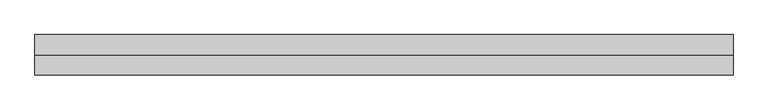
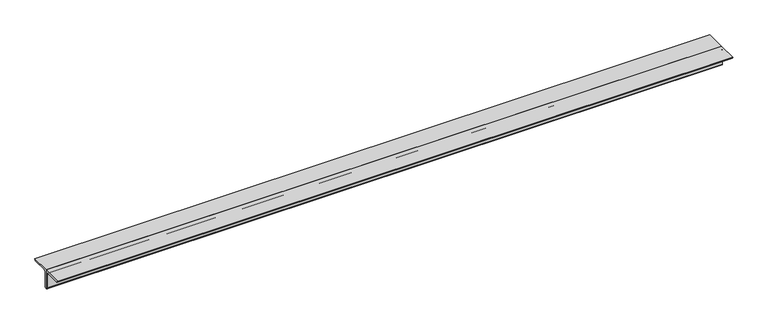
"""IFC4 building model written with IfcOpenShell, lengths in millimetres: member geometry, 0123_Steel Framing_2Ls-KSD3502 : H_SB_AR_S03_2Ls-130x130x12_HBR4."""

import ifcopenshell
import ifcopenshell.guid

model = None  # the IFC model being written
_history = None  # IfcOwnerHistory: only IFC2X3 demands one
_inside = {}  # id of a spatial element -> (the spatial element, [elements in it])
_under = {}  # id of a project, library or spatial element -> (it, [spatial elements below it])
_declared = {}  # id of a project -> (the project, [libraries it declares])
_typed = {}  # id of a type object -> (the type object, [elements of that type])
_made_of = {}  # id of a material, layer set ... -> (it, [elements and type objects made of it])


def new_model(schema):
    """Start an empty IFC model of exactly this schema.

    Asked for "IFC4X3", IfcOpenShell would pick the latest addendum, in which some entities
    have other attributes; the version numbers below select the first issue.
    IFC2X3 requires an IfcOwnerHistory on every rooted entity: one is made here for all.
    """
    global model, _history
    if schema == "IFC4X3":
        model = ifcopenshell.file(schema_version=(4, 3, 0, 0))
    else:
        model = ifcopenshell.file(schema=schema)
    _inside.clear()
    _under.clear()
    _declared.clear()
    _typed.clear()
    _made_of.clear()
    _history = None
    if model.schema == "IFC2X3":
        org = make("IfcOrganization", Name="unknown")
        user = make(
            "IfcPersonAndOrganization",
            ThePerson=make("IfcPerson", FamilyName="unknown"),
            TheOrganization=org,
        )
        app = make(
            "IfcApplication",
            ApplicationDeveloper=org,
            Version="unknown",
            ApplicationFullName="unknown",
            ApplicationIdentifier="unknown",
        )
        _history = make(
            "IfcOwnerHistory",
            OwningUser=user,
            OwningApplication=app,
            ChangeAction="ADDED",
            CreationDate=0,
        )
    return model


def make(cls, **values):
    """One entity of the class cls with the attributes given. An attribute that is None is left unset."""
    return model.create_entity(
        cls, **{name: value for name, value in values.items() if value is not None}
    )


def rooted(cls, **values):
    """An entity with a GlobalId (a new one), such as an element, a storey or a relation."""
    return make(cls, GlobalId=ifcopenshell.guid.new(), OwnerHistory=_history, **values)


def si_unit(unit_type, name, prefix=None):
    """IfcSIUnit, for example si_unit("LENGTHUNIT", "METRE", prefix="MILLI")."""
    return make("IfcSIUnit", UnitType=unit_type, Prefix=prefix, Name=name)


def assignment(units):
    """IfcUnitAssignment: the units of a project."""
    return None if units is None else make("IfcUnitAssignment", Units=units)


def point(xyz):
    """IfcCartesianPoint."""
    return None if xyz is None else make("IfcCartesianPoint", Coordinates=xyz)


def direction(xyz):
    """IfcDirection."""
    return None if xyz is None else make("IfcDirection", DirectionRatios=xyz)


def frame(location, z_axis=None, x_axis=None):
    """IfcAxis2Placement3D, a coordinate frame: its origin and axes. An axis left out is left unset."""
    return make(
        "IfcAxis2Placement3D",
        Location=point(location),
        Axis=direction(z_axis),
        RefDirection=direction(x_axis),
    )


def frame_2d(location, x_axis=None):
    """IfcAxis2Placement2D, a coordinate frame in the plane: its origin and x axis."""
    return make(
        "IfcAxis2Placement2D", Location=point(location), RefDirection=direction(x_axis)
    )


def origin():
    """The frame at (0, 0, 0) with its axes left unset."""
    return frame((0.0, 0.0, 0.0))


def place(relative_to, where):
    """IfcLocalPlacement: puts the frame where relative to a parent placement (None: the world)."""
    return make(
        "IfcLocalPlacement", PlacementRelTo=relative_to, RelativePlacement=where
    )


def context(
    kind, dimensions, precision=None, world=None, true_north=None, identifier=None
):
    """IfcGeometricRepresentationContext, for example the 3D "Model" context."""
    return make(
        "IfcGeometricRepresentationContext",
        ContextIdentifier=identifier,
        ContextType=kind,
        CoordinateSpaceDimension=dimensions,
        Precision=precision,
        WorldCoordinateSystem=world,
        TrueNorth=true_north,
    )


def project(units=None, contexts=None):
    """IfcProject with its units and contexts."""
    return rooted(
        "IfcProject",
        Name="project",
        RepresentationContexts=contexts,
        UnitsInContext=assignment(units),
    )


def spatial(cls, under=None, at=None, **own):
    """A site, building, storey or space (cls), placed at a placement, below another one or the project."""
    s = rooted(cls, ObjectPlacement=at, **own)
    if under is not None:
        _under.setdefault(under.id(), (under, []))[1].append(s)
    return s


def polyline(points):
    """IfcPolyline through the points."""
    return make("IfcPolyline", Points=[point(p) for p in points])


def circle_curve(where, radius):
    """IfcCircle in the frame where."""
    return make("IfcCircle", Position=where, Radius=radius)


def trimmed(basis, trim1, trim2, sense, master):
    """IfcTrimmedCurve: the piece of a basis curve between two trims."""
    return make(
        "IfcTrimmedCurve",
        BasisCurve=basis,
        Trim1=trim1,
        Trim2=trim2,
        SenseAgreement=sense,
        MasterRepresentation=master,
    )


def segment(curve, same_sense, transition):
    """IfcCompositeCurveSegment."""
    return make(
        "IfcCompositeCurveSegment",
        Transition=transition,
        SameSense=same_sense,
        ParentCurve=curve,
    )


def composite_curve(segments, self_intersect=None):
    """IfcCompositeCurve: segments joined end to end."""
    return make("IfcCompositeCurve", Segments=segments, SelfIntersect=self_intersect)


def outline(outer, holes=None, kind="AREA"):
    """IfcArbitraryClosedProfileDef: a profile drawn as a closed curve; with holes, ...WithVoids."""
    if holes is None:
        return make("IfcArbitraryClosedProfileDef", ProfileType=kind, OuterCurve=outer)
    return make(
        "IfcArbitraryProfileDefWithVoids",
        ProfileType=kind,
        OuterCurve=outer,
        InnerCurves=holes,
    )


def extrude(swept, where, along, depth):
    """IfcExtrudedAreaSolid: the profile swept, set in the frame where, extruded along a direction by depth."""
    return make(
        "IfcExtrudedAreaSolid",
        SweptArea=swept,
        Position=where,
        ExtrudedDirection=direction(along),
        Depth=depth,
    )


def shape(context_of_items, identifier, shape_type, items):
    """IfcShapeRepresentation: the items that make up one representation, for example the "Body"."""
    return make(
        "IfcShapeRepresentation",
        ContextOfItems=context_of_items,
        RepresentationIdentifier=identifier,
        RepresentationType=shape_type,
        Items=items,
    )


def source(mapping_origin, context_of_items, identifier, shape_type, items):
    """IfcRepresentationMap: a shape defined once, which mapped items show again and again."""
    return make(
        "IfcRepresentationMap",
        MappingOrigin=mapping_origin,
        MappedRepresentation=shape(context_of_items, identifier, shape_type, items),
    )


def transform(
    local_origin,
    x_axis=None,
    y_axis=None,
    z_axis=None,
    scale=None,
    scale2=None,
    scale3=None,
    uniform=True,
):
    """IfcCartesianTransformationOperator3D, or its non-uniform kind. x_axis, y_axis, z_axis: its Axis1, 2, 3."""
    if uniform:
        return make(
            "IfcCartesianTransformationOperator3D",
            Axis1=direction(x_axis),
            Axis2=direction(y_axis),
            LocalOrigin=point(local_origin),
            Scale=scale,
            Axis3=direction(z_axis),
        )
    return make(
        "IfcCartesianTransformationOperator3DnonUniform",
        Axis1=direction(x_axis),
        Axis2=direction(y_axis),
        LocalOrigin=point(local_origin),
        Scale=scale,
        Axis3=direction(z_axis),
        Scale2=scale2,
        Scale3=scale3,
    )


def mapped(mapping_source, mapping_target):
    """IfcMappedItem: shows the shape of a source again, moved by a transform."""
    return make(
        "IfcMappedItem", MappingSource=mapping_source, MappingTarget=mapping_target
    )


def made_of(thing, what):
    """Note that an element or type object is made of a material, layer set ...; save() writes the relation."""
    if what is not None:
        _made_of.setdefault(what.id(), (what, []))[1].append(thing)
    return thing


def element(
    cls,
    number,
    at=None,
    inside=None,
    cuts=None,
    type_object=None,
    material=None,
    context=None,
    identifier="Body",
    shape_type=None,
    held_by="IfcProductDefinitionShape",
    body=None,
    shapes=None,
    **own,
):
    """One element of the class cls, such as IfcWall. Its Tag is "e" and its number.

    at: its placement. inside: the storey or other place that contains it. cuts: it is an
    opening in that element (IfcRelVoidsElement). A single representation is given by context,
    identifier, shape_type and body (its items); several are given by shapes. held_by: the class
    of the entity that holds the representations. save() writes the other relations.
    """
    e = rooted(cls, Tag="e%d" % number, ObjectPlacement=at, **own)
    if body is not None:
        shapes = [shape(context, identifier, shape_type, body)]
    if shapes is not None:
        e.Representation = make(held_by, Representations=shapes)
    if inside is not None:
        _inside.setdefault(inside.id(), (inside, []))[1].append(e)
    if cuts is not None:
        rooted(
            "IfcRelVoidsElement", RelatingBuildingElement=cuts, RelatedOpeningElement=e
        )
    if type_object is not None:
        _typed.setdefault(type_object.id(), (type_object, []))[1].append(e)
    return made_of(e, material)


def aggregate(whole, parts):
    """IfcRelAggregates: a whole, such as a stair, and the parts it consists of."""
    return rooted("IfcRelAggregates", RelatingObject=whole, RelatedObjects=parts)


def save(model, path):
    """Write the relations noted so far, then the file.

    IfcRelAggregates (storeys below a building ...), IfcRelContainedInSpatialStructure (elements
    in a storey), IfcRelDefinesByType, IfcRelAssociatesMaterial and IfcRelDeclares: one each for
    every whole, place, type object, material and project.
    """
    for whole, parts in _under.values():
        aggregate(whole, parts)
    for where, things in _inside.values():
        rooted(
            "IfcRelContainedInSpatialStructure",
            RelatedElements=things,
            RelatingStructure=where,
        )
    for kind, things in _typed.values():
        rooted("IfcRelDefinesByType", RelatedObjects=things, RelatingType=kind)
    for what, things in _made_of.values():
        rooted("IfcRelAssociatesMaterial", RelatedObjects=things, RelatingMaterial=what)
    for by, libraries in _declared.values():
        rooted("IfcRelDeclares", RelatingContext=by, RelatedDefinitions=libraries)
    model.write(path)


def member_0d683159(model_context):
    return source(origin(), model_context, "Body", "SweptSolid", [
        extrude(outline(composite_curve([segment(polyline([(0.0, 36.4), (130.0, 36.4)]), True, "CONTINUOUS"), segment(trimmed(circle_curve(frame_2d((118.0, 36.4)), 12.0), [point((130.0, 36.4))], [point((118.0, 24.4))], False, "CARTESIAN"), True, "CONTINUOUS"), segment(polyline([(118.0, 24.4), (24.0, 24.4)]), True, "CONTINUOUS"), segment(trimmed(circle_curve(frame_2d((24.0, 12.4)), 12.0), [point((24.0, 24.4))], [point((12.0, 12.4))], True, "CARTESIAN"), True, "CONTINUOUS"), segment(polyline([(12.0, 12.4), (12.0, -81.6)]), True, "CONTINUOUS"), segment(trimmed(circle_curve(frame_2d((0.0, -81.6)), 12.0), [point((12.0, -81.6))], [point((0.0, -93.6))], False, "CARTESIAN"), True, "CONTINUOUS"), segment(polyline([(0.0, -93.6), (0.0, 36.4)]), True, "CONTINUOUS")], self_intersect=False)), frame((-2372.2356031, 0.0, 0.0), z_axis=(1.0, 0.0, 0.0), x_axis=(0.0, 1.0, 0.0)), (0.0, 0.0, 1.0), 4480.8559461),
        extrude(outline(composite_curve([segment(polyline([(0.0, 36.4), (0.0, -93.6)]), True, "CONTINUOUS"), segment(trimmed(circle_curve(frame_2d((0.0, -81.6)), 12.0), [point((0.0, -93.6))], [point((-12.0, -81.6))], False, "CARTESIAN"), True, "CONTINUOUS"), segment(polyline([(-12.0, -81.6), (-12.0, 12.4)]), True, "CONTINUOUS"), segment(trimmed(circle_curve(frame_2d((-24.0, 12.4)), 12.0), [point((-12.0, 12.4))], [point((-24.0, 24.4))], True, "CARTESIAN"), True, "CONTINUOUS"), segment(polyline([(-24.0, 24.4), (-118.0, 24.4)]), True, "CONTINUOUS"), segment(trimmed(circle_curve(frame_2d((-118.0, 36.4)), 12.0), [point((-118.0, 24.4))], [point((-130.0, 36.4))], False, "CARTESIAN"), True, "CONTINUOUS"), segment(polyline([(-130.0, 36.4), (0.0, 36.4)]), True, "CONTINUOUS")], self_intersect=False)), frame((-2372.2356031, 0.0, 0.0), z_axis=(1.0, 0.0, 0.0), x_axis=(0.0, 1.0, 0.0)), (0.0, 0.0, 1.0), 4480.8559461),
    ])


if __name__ == "__main__":
    model = new_model("IFC4")
    model_context = context("Model", 3, world=origin())
    ifc_project = project(units=[si_unit("LENGTHUNIT", "METRE", prefix="MILLI")], contexts=[model_context])
    site = spatial("IfcSite", under=ifc_project)
    building = spatial("IfcBuilding", under=site)
    placement = place(None, origin())
    member_shape = member_0d683159(model_context)
    element("IfcMember", 1, ObjectType="0123_Steel Framing_2Ls-KSD3502 : H_SB_AR_S03_2Ls-130x130x12_HBR4", at=placement, inside=building, context=model_context, shape_type="MappedRepresentation", body=[
        mapped(member_shape, transform((0.0, 0.0, 0.0), x_axis=(1.0, 0.0, 0.0), y_axis=(0.0, 1.0, 0.0), z_axis=(0.0, 0.0, 1.0))),
    ])
    save(model, "model.ifc")

# Revit data of these elements
# Type "0123_Steel Framing_2Ls-KSD3502 : H_SB_AR_S03_2Ls-130x130x12_HBR4"
#   Type Mark = "HBR4"
#   Assembly Code = "B10"
#   Legs = "SLBB"
#   W = 8.97
#   Perimeter = 1.04 m²/m
#   Nominal Weight = 46.80 kgf/m
#   Length [instance default] = 1000 mm
#   Space = 0 mm
#   b = 130 mm
#   d = 130 mm
#   t = 12 mm
#   y = 36.4 mm
#   A = 0.005952 m²
#   Structural Material [instance default] = Steel ASTM A36
# Element 1 (IfcMember, "0123_Steel Framing_2Ls-KSD3502 : H_SB_AR_S03_2Ls-130x130x12_HBR4")
#   Materials on its faces: "Steel ASTM A36"
# Materials
#   "Steel ASTM A36": class "Metal", colour RGB 199 199 199, transparency 0, Description = "Structural steel, ASTM A36 Grade B, mill finish", Cost = 0
